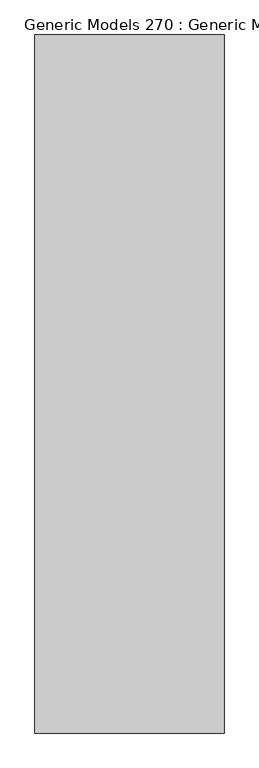
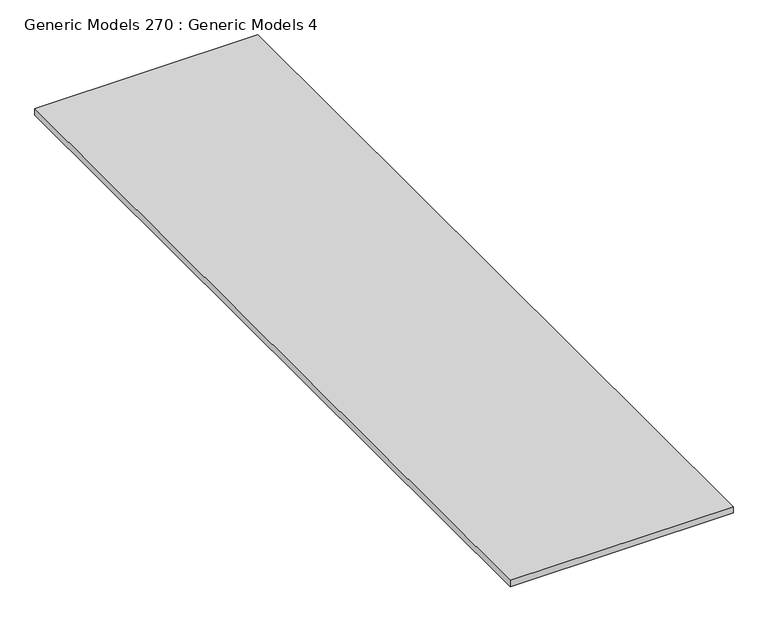
"""IFC4 building model written with IfcOpenShell, lengths in millimetres: proxy geometry, Generic Models 270 : Generic Models 4."""

from ifc_helpers import new_model, si_unit, frame, origin, place, context, project, spatial, polyline, outline, extrude, source, transform, mapped, element, save


def generic_models_270_generic_models_4_657d7f01(model_context):
    return source(origin(), model_context, "Body", "SweptSolid", [
        extrude(outline(polyline([(5023.9999648, -5493.3230338), (1625.4263704, -5493.3230338), (1625.4263704, 7054.2769662), (5023.9999648, 7054.2769662), (5023.9999648, -5493.3230338)])), frame((0.0, 0.0, 123138.946), z_axis=(0.0, 0.0, 1.0), x_axis=(1.0, 0.0, 0.0)), (0.0, 0.0, 1.0), 101.6),
    ])


if __name__ == "__main__":
    model = new_model("IFC4")
    model_context = context("Model", 3, world=origin())
    ifc_project = project(units=[si_unit("LENGTHUNIT", "METRE", prefix="MILLI")], contexts=[model_context])
    site = spatial("IfcSite", under=ifc_project)
    building = spatial("IfcBuilding", under=site)
    placement = place(None, origin())
    generic_models_270_generic_models_4_shape = generic_models_270_generic_models_4_657d7f01(model_context)
    element("IfcBuildingElementProxy", 1, Name="Generic Models 270 : Generic Models 4", ObjectType="Generic Models 270 : Generic Models 4", at=placement, inside=building, context=model_context, shape_type="MappedRepresentation", body=[
        mapped(generic_models_270_generic_models_4_shape, transform((0.0, 0.0, 0.0), x_axis=(1.0, 0.0, 0.0), y_axis=(0.0, 1.0, 0.0), z_axis=(0.0, 0.0, 1.0))),
    ])
    save(model, "model.ifc")

# Revit data of these elements
# Element 1 (IfcBuildingElementProxy, "Generic Models 270 : Generic Models 4")
#   Materials on its faces: "_4\" MIN. CRUSHED GRAVEL (NO FINES)"
# Materials
#   "_4\" MIN. CRUSHED GRAVEL (NO FINES)": class "Generic", colour RGB 122 131 148, transparency 0, Cost = 0
